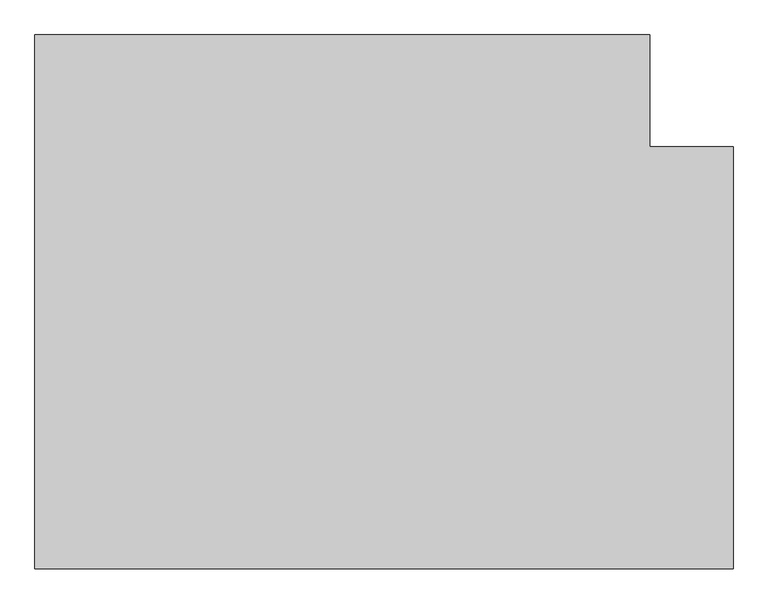
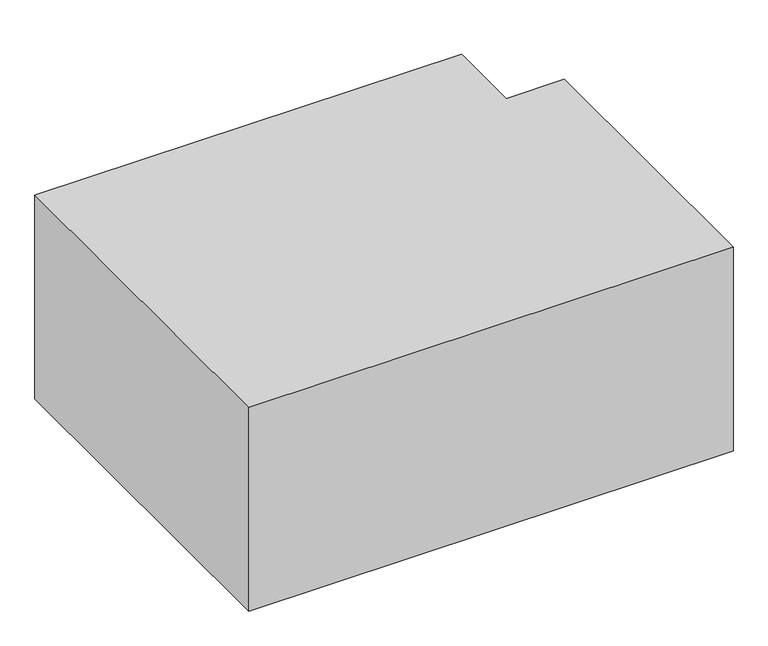
"""IFC4 building model written with IfcOpenShell, lengths in millimetres: proxy geometry, 0_3d."""

from ifc_helpers import new_model, si_unit, origin, origin_with_axes, place, context, project, spatial, polyline, outline, extrude, source, transform, mapped, element, save


def generic_models_f878335a(model_context):
    return source(origin(), model_context, "Body", "SweptSolid", [
        extrude(outline(polyline([(5620.0, 3397.8619019), (5620.0, 0.0), (0.0, 0.0), (0.0, 4297.8619019), (4950.0, 4297.8619019), (4950.0, 3397.8619019), (5620.0, 3397.8619019)])), origin_with_axes(), (0.0, 0.0, 1.0), 2500.0),
    ])


if __name__ == "__main__":
    model = new_model("IFC4")
    model_context = context("Model", 3, world=origin())
    ifc_project = project(units=[si_unit("LENGTHUNIT", "METRE", prefix="MILLI")], contexts=[model_context])
    site = spatial("IfcSite", under=ifc_project)
    building = spatial("IfcBuilding", under=site)
    placement = place(None, origin())
    generic_models_shape = generic_models_f878335a(model_context)
    element("IfcBuildingElementProxy", 1, Name="0_3d", ObjectType="0_3d", at=placement, inside=building, context=model_context, shape_type="MappedRepresentation", body=[
        mapped(generic_models_shape, transform((0.0, 0.0, 0.0), x_axis=(1.0, 0.0, 0.0), y_axis=(0.0, 1.0, 0.0), z_axis=(0.0, 0.0, 1.0))),
    ])
    save(model, "model.ifc")

# Revit data of these elements
# Element 1 (IfcBuildingElementProxy, "0_3d")
#   Materials on its faces: "*1"
# Materials
#   "*1": class "Unassigned", colour RGB 175 175 175, transparency 0
